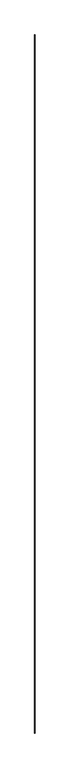
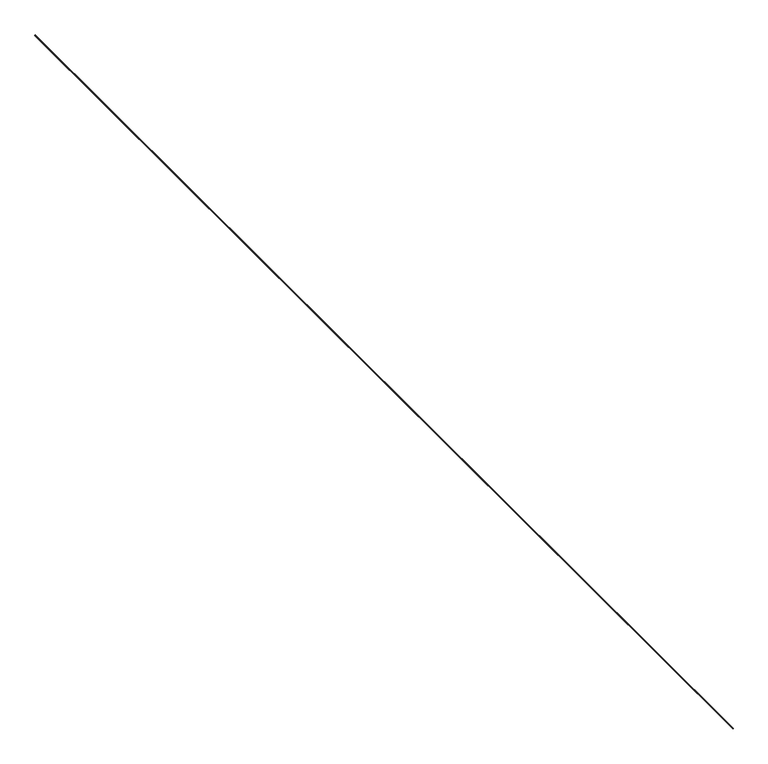
"""IFC4 building model written with IfcOpenShell, lengths in millimetres: proxy geometry, Generic Models 7:Generic Models 1:1:Generic Models 1:1 : Generic Models 7:Generic Models 1:337419:33 : Generic Models 7:Generic Models 1:1:Generic Models 1:1 : Generic Models 7:Generic Models 1:337419:306201."""

from ifc_helpers import new_model, si_unit, frame, origin, place, context, project, spatial, polyline, outline, extrude, source, transform, mapped, element, save


def generic_models_bdb8fa14(model_context):
    return source(origin(), model_context, "Body", "SweptSolid", [
        extrude(outline(polyline([(-11.7361843, 667369.5117239), (-10.0156223, 667370.2843591), (-7.396472, 667372.45133), (-6.195765, 667375.1518255), (-6.6013407, 667377.9633781), (-8.5497508, 667380.4461463), (-11.7361843, 667382.2117239), (0.0, 667382.2117239), (-0.7548172, 667380.2801975), (-1.3821894, 667375.8617239), (-0.7548172, 667371.4432504), (0.0, 667369.5117239), (-11.7361843, 667369.5117239)])), frame((0.0, -507566.8760392, 0.0), z_axis=(0.0, 1.0, 0.0), x_axis=(0.0, 0.0, 1.0)), (0.0, 0.0, 1.0), 38252.9096551),
        extrude(outline(polyline([(-18.5829513, 667369.6709317), (-22.4021798, 667370.897094), (-25.0451679, 667373.1065622), (-25.9884394, 667375.8617239), (-25.0451679, 667378.6168857), (-22.4021798, 667380.8263538), (-18.5829513, 667382.0525162), (-16.4634394, 667382.2117239), (-14.3439275, 667382.0525162), (-10.524699, 667380.8263538), (-7.8817109, 667378.6168857), (-6.9384394, 667375.8617239), (-7.8817109, 667373.1065622), (-10.524699, 667370.897094), (-14.3439275, 667369.6709317), (-16.4634394, 667369.5117239), (-18.5829513, 667369.6709317)])), frame((0.0, -507566.8760392, 0.0), z_axis=(0.0, 1.0, 0.0), x_axis=(0.0, 0.0, 1.0)), (0.0, 0.0, 1.0), 38252.9096551),
    ])


if __name__ == "__main__":
    model = new_model("IFC4")
    model_context = context("Model", 3, world=origin())
    ifc_project = project(units=[si_unit("LENGTHUNIT", "METRE", prefix="MILLI")], contexts=[model_context])
    site = spatial("IfcSite", under=ifc_project)
    building = spatial("IfcBuilding", under=site)
    placement = place(None, origin())
    generic_models_shape = generic_models_bdb8fa14(model_context)
    element("IfcBuildingElementProxy", 1, Name="Generic Models 7:Generic Models 1:1:Generic Models 1:1 : Generic Models 7:Generic Models 1:337419:33 : Generic Models 7:Generic Models 1:1:Generic Models 1:1 : Generic Models 7:Generic Models 1:337419:306201", ObjectType="Generic Models 7:Generic Models 1:1:Generic Models 1:1 : Generic Models 7:Generic Models 1:337419:33 : Generic Models 7:Generic Models 1:1:Generic Models 1:1 : Generic Models 7:Generic Models 1:337419:306201", at=placement, inside=building, context=model_context, shape_type="MappedRepresentation", body=[
        mapped(generic_models_shape, transform((0.0, 0.0, 0.0), x_axis=(1.0, 0.0, 0.0), y_axis=(0.0, 1.0, 0.0), z_axis=(0.0, 0.0, 1.0))),
    ])
    save(model, "model.ifc")

# Revit data of these elements
# Type "Generic Models 7:Generic Models 1:1:Generic Models 1:1 : Generic Models 7:Generic Models 1:337419:33 : Generic Models 7:Generic Models 1:1:Generic Models 1:1 : Generic Models 7:Generic Models 1:337419:306201"
#   NameOverride = "Generic Models 7:Generic Models 1:1:Generic Models 1:1 : Generic Models 7:Generic Models 1:337419:306201"
#   ObjectTypeOverride = "Generic Models 1:1 : Generic Models 7:Generic Models 1:337419"
#   Reference = "Generic Models 1"
#   Tag = "306201"
# Element 1 (IfcBuildingElementProxy, "Generic Models 7:Generic Models 1:1:Generic Models 1:1 : Generic Models 7:Generic Models 1:337419:33 : Generic Models 7:Generic Models 1:1:Generic Models 1:1 : Generic Models 7:Generic Models 1:337419:306201")
#   Materials on its faces: "SEMI-RIGID EPOXY SEALANT W/ BACKROD (REMOVE TEMP. JOINT FORM)"
# Materials
#   "SEMI-RIGID EPOXY SEALANT W/ BACKROD (REMOVE TEMP. JOINT FORM)": class "Unassigned", colour RGB 120 120 120, transparency 0, Cost = 0
